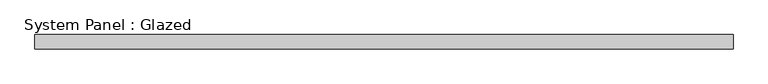
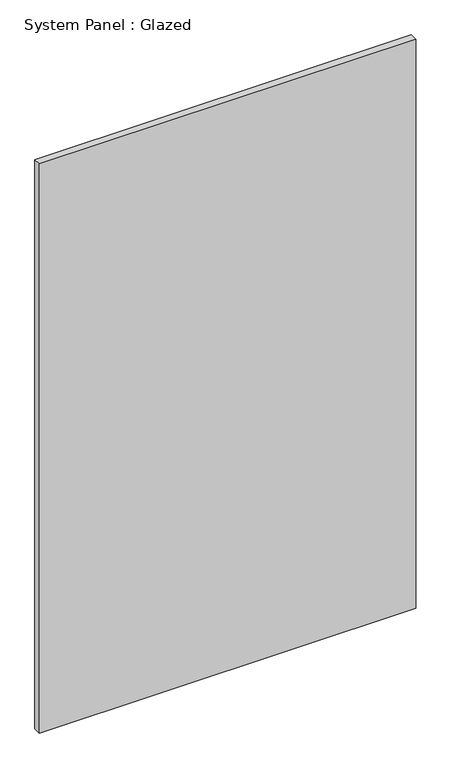
"""IFC4 building model written with IfcOpenShell, lengths in millimetres: plate geometry, System Panel : Glazed."""

from ifc_helpers import new_model, si_unit, origin, origin_with_axes, place, context, project, spatial, polyline, outline, extrude, source, transform, mapped, element, save


def system_panel_glazed_5cc509e3(model_context):
    return source(origin(), model_context, "Body", "SweptSolid", [
        extrude(outline(polyline([(624.6304833, 19.05), (-624.6304833, 19.05), (-624.6304833, 44.45), (624.6304833, 44.45), (624.6304833, 19.05)])), origin_with_axes(), (0.0, 0.0, 1.0), 1996.44),
    ])


if __name__ == "__main__":
    model = new_model("IFC4")
    model_context = context("Model", 3, world=origin())
    ifc_project = project(units=[si_unit("LENGTHUNIT", "METRE", prefix="MILLI")], contexts=[model_context])
    site = spatial("IfcSite", under=ifc_project)
    building = spatial("IfcBuilding", under=site)
    placement = place(None, origin())
    system_panel_glazed_shape = system_panel_glazed_5cc509e3(model_context)
    element("IfcPlate", 1, ObjectType="System Panel : Glazed", at=placement, inside=building, context=model_context, shape_type="MappedRepresentation", body=[
        mapped(system_panel_glazed_shape, transform((0.0, 0.0, 0.0), x_axis=(1.0, 0.0, 0.0), y_axis=(0.0, 1.0, 0.0), z_axis=(0.0, 0.0, 1.0))),
    ])
    save(model, "model.ifc")

# Revit data of these elements
# Type "System Panel : Glazed"
#   Construction Type Id = "GSP4R"
#   Analytic Construction = "1/8 in Pilkington single glazing"
#   Visual Light Transmittance = 0.9
#   Solar Heat Gain Coefficient = 0.86
#   Heat Transfer Coefficient (U) = 1.18115 BTU/(h·ft²·°F)
#   Define Thermal Properties by = 1
# Element 1 (IfcPlate, "System Panel : Glazed")
#   Materials on its faces: "Glass"
# Materials
#   "Glass": class "Glass", colour RGB 0 128 192, transparency 0.75, Description = "Soda Lime Glass", Cost = 0
